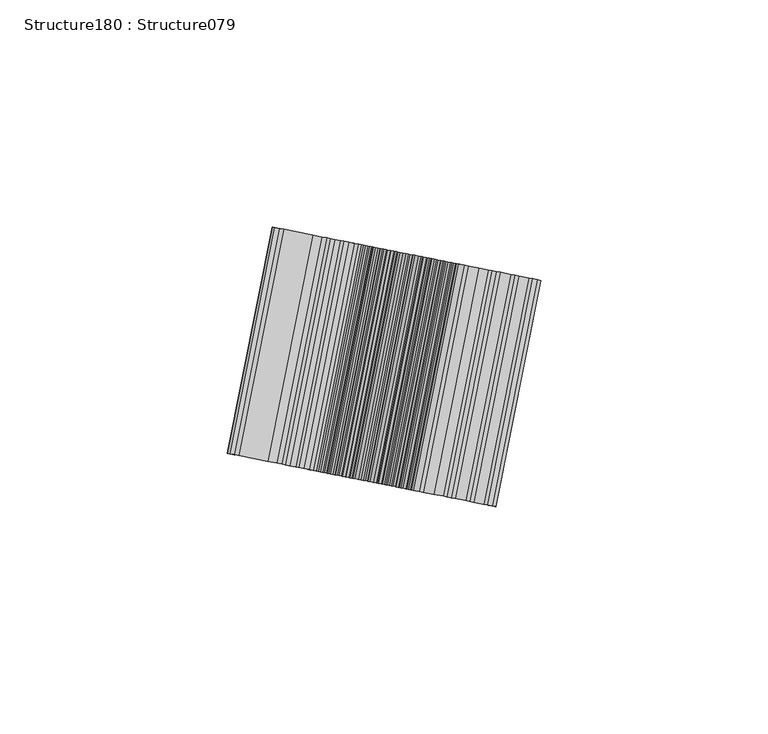
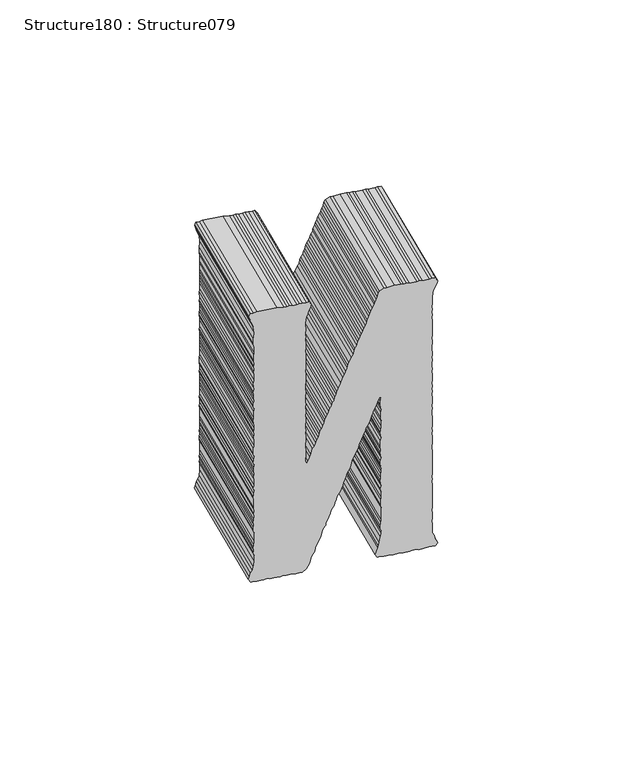
"""IFC4 building model written with IfcOpenShell, lengths in millimetres: proxy geometry, Structure180 : Structure079."""

from ifc_helpers import new_model, si_unit, frame, origin, place, context, project, spatial, polyline, outline, extrude, source, transform, mapped, element, save


def structure180_structure079_712ac3f3(model_context):
    return source(origin(), model_context, "Body", "SweptSolid", [
        extrude(outline(polyline([(1.8366799, 0.0), (3.1719919, 0.2053232), (3.9678799, 0.2224656), (6.1339986, 0.7044793), (7.2017339, -0.1002347), (6.923545, -1.1141612), (6.9103347, -2.1601811), (6.6008944, -4.347663), (6.6194392, -5.1387183), (6.4560722, -6.2935846), (6.200152, -7.1805736), (6.164673, -8.353531), (5.8919629, -10.2813618), (5.504575, -11.1450816), (5.322519, -12.4320636), (5.4731794, -13.2418079), (5.3278037, -14.2694911), (4.776401, -16.2926574), (4.4850018, -18.3526037), (3.4817959, -18.994451), (2.4123488, -18.1891354), (1.5488816, -17.802502), (0.6787273, -17.4199537), (-0.4031239, -16.7429712), (-2.5708599, -16.3015648), (-3.6179366, -16.2882051), (-4.4817562, -15.9015218), (-5.5316583, -15.8827314), (-7.7145603, -15.573939), (-8.6005919, -15.318873), (-9.646971, -15.3005809), (-13.7622836, -14.7184305), (-14.8072465, -14.7053698), (-15.8412712, -14.5590971), (-16.8492085, -14.2817553), (-18.0093595, -14.1176408), (-19.0176422, -13.8452812), (-20.0827102, -13.9591049), (-20.8239266, -13.589765), (-22.015121, -13.6857468), (-23.1509461, -13.390314), (-24.0757719, -13.394248), (-27.2905847, -12.9394819), (-28.3002834, -12.6618909), (-29.3265574, -12.5167146), (-30.11962, -12.5392877), (-31.369217, -12.0980324), (-33.4665482, -12.0658325), (-34.4928222, -11.9206562), (-35.3742807, -11.6612061), (-36.5167928, -11.3698585), (-37.5628196, -11.3516162), (-38.4453282, -11.0970486), (-39.363467, -11.0968974), (-40.5405456, -11.0651477), (-42.5969688, -10.7742469), (-43.5925517, -10.3689245), (-44.6191778, -10.2236983), (-45.6838937, -10.3375718), (-46.5473609, -9.9509383), (-47.870671, -10.0282311), (-48.6260031, -9.7866228), (-49.6713184, -9.7735123), (-50.7947892, -9.3500988), (-51.9916205, -9.4452833), (-52.7233245, -9.077289), (-53.9145189, -9.1732708), (-54.7818616, -8.7860892), (-56.1069332, -8.8631328), (-58.1672318, -8.5716838), (-59.0250621, -8.1858477), (-60.0943579, -8.2990733), (-61.0857131, -7.8943489), (-61.989736, -7.7664662), (-63.3091707, -7.8443072), (-64.3005258, -7.4395828), (-65.1151027, -7.5888408), (-66.1230399, -7.311499), (-67.2592105, -7.0210484), (-68.4193615, -6.8569339), (-69.3565418, -6.9888485), (-70.5114082, -6.8254816), (-71.248749, -6.4566899), (-72.4268914, -6.4197587), (-73.4774913, -6.4059007), (-74.6320055, -6.2425836), (-75.382053, -6.0017227), (-76.673615, -5.8190189), (-77.7189303, -5.8059084), (-78.7109901, -5.4010843), (-79.7608922, -5.3822939), (-80.6391731, -5.1283243), (-81.7077643, -5.2416496), (-82.8298258, -4.8184355), (-83.6348904, -4.9690391), (-84.9045926, -4.6546681), (-85.695189, -4.6775901), (-88.0278455, -4.4773417), (-88.9646734, -4.6093061), (-90.210194, -5.0867878), (-91.0208956, -5.2365939), (-92.1011932, -5.4733199), (-93.1586381, -4.5399738), (-93.1207497, -3.3626855), (-92.7520508, -2.6310813), (-92.4419626, -0.4390193), (-92.5745818, 0.4982605), (-92.1872438, 1.3616281), (-91.8598122, 3.6762933), (-91.9924812, 4.6132209), (-91.587102, 5.604124), (-91.7377623, 6.4138683), (-91.4463133, 8.4741669), (-90.858928, 10.7516999), (-90.7315437, 11.6521997), (-89.7588844, 12.9570716), (-88.9361808, 13.2349082), (-87.6075862, 13.3114535), (-86.6587493, 13.5664164), (-85.7042825, 13.8256138), (-84.8931789, 13.9757224), (-83.775553, 14.4763272), (-82.5614281, 14.6937625), (-81.6062565, 14.9528603), (-80.6633896, 15.0843297), (-79.4362126, 15.4346781), (-78.6501893, 15.4532159), (-77.5449108, 15.8208079), (-76.462154, 16.0622168), (-75.3808561, 16.3034728), (-74.534172, 16.7076456), (-73.5973441, 16.8396099), (-72.5104094, 17.0800685), (-71.6883537, 17.3533251), (-70.4908177, 17.4484099), (-69.4996705, 17.9669062), (-68.5635403, 18.0939382), (-67.3684206, 18.1897241), (-66.2493787, 18.6850975), (-64.4672759, 19.2214339), (-63.510293, 19.4806349), (-62.4663801, 19.4626917), (-61.3649772, 19.8308319), (-60.1522683, 20.0534986), (-59.1790557, 20.4401319), (-57.1595208, 20.813153), (-55.3756564, 21.3492401), (-54.1632432, 21.567277), (-53.2264153, 21.6992414), (-52.2712438, 21.9583392), (-51.0789855, 22.0491394), (-50.3414505, 22.603871), (-49.2971852, 22.585878), (-48.3063834, 23.0993922), (-47.1095521, 23.1945765), (-46.0042238, 23.5625208), (-45.0532801, 23.8222168), (-44.0981086, 24.0813146), (-43.3078576, 24.0992543), (-41.9482196, 24.4358958), (-40.9757116, 24.8226288), (-40.0205401, 25.0817266), (-38.9505328, 25.1898204), (-37.8872262, 25.3038931), (-37.0641205, 25.5820323), (-35.9782357, 25.8176085), (-34.8771851, 26.1857985), (-34.0315648, 26.5951527), (-32.0246798, 26.8355632), (-31.0754975, 27.0955083), (-29.7162049, 27.4271675), (-28.755699, 27.6858701), (-29.9749504, 28.3822892), (-32.0662924, 28.413642), (-34.1269434, 28.7051408), (-34.8625227, 29.0736832), (-36.0187983, 29.2372495), (-37.0630636, 29.2552425), (-38.22709, 29.4199053), (-39.2741669, 29.433265), (-40.0058708, 29.8012592), (-41.0748143, 29.6879839), (-42.0665217, 30.092758), (-43.098785, 30.2387816), (-44.289627, 30.14275), (-45.1714379, 30.4022499), (-46.4397241, 30.7113895), (-47.2320888, 30.6937488), (-48.2731764, 30.7062613), (-49.4008748, 31.1302727), (-50.4469016, 31.1485149), (-51.4555365, 31.4209243), (-53.5158352, 31.7123733), (-54.5844263, 31.5990481), (-56.5985323, 32.1484504), (-57.376429, 32.2584913), (-58.4418493, 32.1447176), (-59.7094377, 32.4587895), (-60.5003864, 32.4359175), (-61.5231373, 32.5805954), (-62.778019, 33.0225981), (-63.5834359, 32.8720444), (-65.6440868, 33.1635433), (-66.9116752, 33.4776151), (-68.9719739, 33.7690641), (-69.8488455, 34.0228343), (-70.9195505, 33.9098082), (-71.801009, 34.1692583), (-72.9555232, 34.3325754), (-74.1015584, 34.6244214), (-75.1479374, 34.6427134), (-75.9022058, 34.8791403), (-78.2475621, 34.9464258), (-79.2452588, 35.3520472), (-80.2711804, 35.4971736), (-82.2586151, 35.3840994), (-83.4696121, 35.1608312), (-84.40997, 35.0343972), (-85.6367947, 34.683999), (-86.7195018, 34.4429424), (-87.7897033, 35.2480053), (-87.5340788, 36.1303644), (-87.3520727, 37.416994), (-87.3342395, 38.4677503), (-86.9711775, 39.2001521), (-86.7891714, 40.4867817), (-86.8981623, 41.5504475), (-86.5344526, 42.2874292), (-86.3883792, 43.3200446), (-86.3520443, 45.4110413), (-85.4425121, 51.8406667), (-85.0420721, 52.8372996), (-85.0228229, 53.8828246), (-83.9355358, 54.1232334), (-82.7042823, 53.5548448), (-81.9483022, 53.3178165), (-80.8660987, 52.6407842), (-79.8927349, 52.1088765), (-77.7426378, 51.540237), (-75.6456589, 51.5080868), (-73.7185328, 51.2354763), (-72.7233023, 50.8302038), (-70.5404003, 50.5214114), (-69.7476901, 50.5440342), (-67.5556282, 50.233946), (-66.5515663, 49.9571525), (-65.5062512, 49.9440419), (-64.6191556, 49.6837945), (-63.5738403, 49.6706839), (-62.4323783, 49.3744538), (-60.3777166, 49.0838022), (-59.3066593, 49.1967785), (-57.288678, 48.6468281), (-56.2200868, 48.7601532), (-55.0832117, 48.469603), (-54.1777794, 48.3415209), (-53.041602, 48.0460384), (-52.2365374, 48.1966419), (-50.9442707, 48.0138384), (-50.0811559, 47.6272549), (-49.0358406, 47.6141443), (-46.8473017, 47.3045545), (-45.9252875, 47.303855), (-44.7887646, 47.0133546), (-44.0390694, 46.7725438), (-43.0071585, 46.6265701), (-41.8318415, 46.5950695), (-40.9500307, 46.3355696), (-39.7733044, 46.3038697), (-38.6314901, 46.0075898), (-36.5771807, 45.716988), (-35.6400005, 45.8489025), (-33.5797019, 45.5574535), (-32.7102453, 45.1699729), (-31.4109159, 45.1209296), (-30.6245403, 45.1394175), (-29.6289575, 44.7340951), (-28.5822329, 44.7207852), (-27.5538452, 44.5753099), (-26.2823814, 44.2606898), (-25.4953081, 44.2841101), (-24.2256058, 43.9697392), (-22.1670688, 43.6785394), (-21.2298885, 43.8104539), (-20.3664213, 43.4238205), (-19.059341, 43.3736808), (-18.0094388, 43.3548903), (-17.1329196, 43.10117), (-13.9177545, 42.646354), (-13.030659, 42.3861065), (-11.8574559, 42.354905), (-11.1017713, 42.1132469), (-9.7968049, 42.0634061), (-9.0104293, 42.0818941), (-7.7421432, 41.7727545), (-6.8180151, 41.771756), (-5.7917412, 41.6265798), (-4.9282739, 41.2399464), (-1.7131088, 40.7851304), (-0.5342688, 40.7531315), (0.3782332, 40.7537777), (1.5263822, 40.4616327), (2.3127577, 40.4801206), (3.4341147, 40.0570063), (5.6226535, 39.7474165), (7.4599812, 39.7519964), (8.7952933, 39.9573198), (9.6458529, 40.3609442), (10.9833286, 40.5663207), (11.7933325, 40.7111946), (12.8430266, 39.778945), (12.7156921, 38.8787974), (12.715498, 37.9552742), (12.4062518, 36.6913155), (12.2789172, 35.7911679), (11.982737, 34.6500582), (12.1333973, 33.8403139), (11.8234534, 32.5714229), (11.6606399, 30.4983179), (11.273252, 29.634598), (11.3878799, 28.5701349), (10.9638616, 27.4474684), (10.8544685, 26.6741518), (10.9691462, 25.610041), (10.6771936, 24.4683332), (10.5498093, 23.5678333), (9.4634279, 22.4091362), (8.5124343, 22.149088), (7.3955061, 21.6534156), (6.4713781, 21.654414), (5.2621923, 21.431249), (4.2833428, 21.0454131), (3.3161692, 20.6582847), (2.1193378, 20.5631003), (1.0144118, 20.1954585), (-0.8952764, 19.6768109), (-1.8465726, 19.4171649), (-2.6424604, 19.4000225), (-3.9777725, 19.1946993), (-4.8065152, 18.9173575), (-5.9237956, 18.421735), (-6.8426322, 18.4169539), (-7.9493198, 18.0495611), (-8.9041889, 17.7900612), (-9.8713623, 17.4029329), (-11.0533802, 17.4404124), (-11.8951251, 17.0305099), (-13.000101, 16.6625158), (-13.9147167, 16.6621686), (-15.0154151, 16.2939287), (-15.8243551, 16.1438733), (-16.9067666, 15.9074465), (-17.9021415, 15.3895483), (-19.94002, 14.8893937), (-20.9846376, 14.9074366), (-22.0857381, 14.5388942), (-22.9183063, 14.2624531), (-24.2373886, 14.1845623), (-26.0371803, 13.5206404), (-27.1258766, 13.280431), (-28.0443677, 13.2806321), (-29.2535535, 13.057467), (-30.0798369, 12.7848084), (-31.1812329, 12.4116362), (-31.990173, 12.2615809), (-33.2413305, 11.7848964), (-34.2873573, 11.8031386), (-35.3923332, 11.4351445), (-36.3235242, 11.3023827), (-37.4284502, 10.9347408), (-39.4663786, 10.4342341), (-40.4025087, 10.307202), (-41.2622449, 9.7701163), (-42.2224055, 9.5163959), (-43.3033511, 9.2750901), (-44.3722945, 9.1618148), (-45.1766614, 9.0161435), (-46.3861926, 8.7879963), (-47.5112736, 8.2931179), (-48.4484538, 8.1612034), (-49.2746874, 7.8888971), (-50.3573944, 7.6478403), (-51.4623703, 7.2798462), (-50.4487962, 7.0017071), (-49.5334827, 7.0069865), (-48.2419206, 6.8242826), (-47.3601098, 6.5647827), (-46.3514748, 6.2923733), (-45.4333359, 6.2922221), (-43.3726851, 6.0007233), (-42.1043989, 5.6915837), (-40.3037515, 5.4368648), (-38.9977212, 5.3818426), (-38.2106479, 5.4052629), (-37.1970738, 5.1271238), (-36.060551, 4.8366234), (-34.9954828, 4.9504469), (-32.8090579, 4.6411561), (-31.7954837, 4.363017), (-30.8766472, 4.3677981), (-29.740822, 4.0723654), (-28.8526765, 3.8170004), (-27.7897223, 3.9311229), (-26.6330943, 3.7675068), (-25.7477604, 3.5075085), (-24.8694795, 3.2535389), (-23.8372163, 3.1075154), (-22.9190774, 3.1073642), (-21.6324477, 2.925358), (-20.5857232, 2.9120481), (-19.577786, 2.6347064), (-18.6899928, 2.3793912), (-17.6249247, 2.4932147), (-16.5070909, 2.0705988), (-14.4485539, 1.779399), (-13.5300626, 1.7791979), (-11.469764, 1.4877489), (-10.5876078, 1.2332311), (-6.2122917, 0.6143007), (-5.2997897, 0.6149468), (-4.1149604, 0.5821006), (-3.2204497, 0.4555635), (-2.3513456, 0.0681328), (-1.3247193, -0.0770934), (0.0, 0.0), (1.8366799, 0.0)])), frame((-2150.5465494, 234895.2724928, 393.6733864), z_axis=(0.19466222296394117, 0.9808703374813293, 0.0), x_axis=(-0.1373857309712728, 0.027265389493846895, -0.9901422925323602)), (0.0, 0.0, 1.0), 50.8),
    ])


if __name__ == "__main__":
    model = new_model("IFC4")
    model_context = context("Model", 3, world=origin())
    ifc_project = project(units=[si_unit("LENGTHUNIT", "METRE", prefix="MILLI")], contexts=[model_context])
    site = spatial("IfcSite", under=ifc_project)
    building = spatial("IfcBuilding", under=site)
    placement = place(None, origin())
    structure180_structure079_shape = structure180_structure079_712ac3f3(model_context)
    element("IfcBuildingElementProxy", 1, Name="Structure180 : Structure079", ObjectType="Structure180 : Structure079", at=placement, inside=building, context=model_context, shape_type="MappedRepresentation", body=[
        mapped(structure180_structure079_shape, transform((0.0, 0.0, 0.0), x_axis=(1.0, 0.0, 0.0), y_axis=(0.0, 1.0, 0.0), z_axis=(0.0, 0.0, 1.0))),
    ])
    save(model, "model.ifc")

# Revit data of these elements
# Type "Structure180 : Structure079"
#   NameOverride = "Structure079"
# Element 1 (IfcBuildingElementProxy, "Structure180 : Structure079")
#   Materials on its faces: "BRUSHED ALUMINUM LETTERING"
# Materials
#   "BRUSHED ALUMINUM LETTERING": class "Unassigned", colour RGB 169 181 186, transparency 0, Cost = 0
